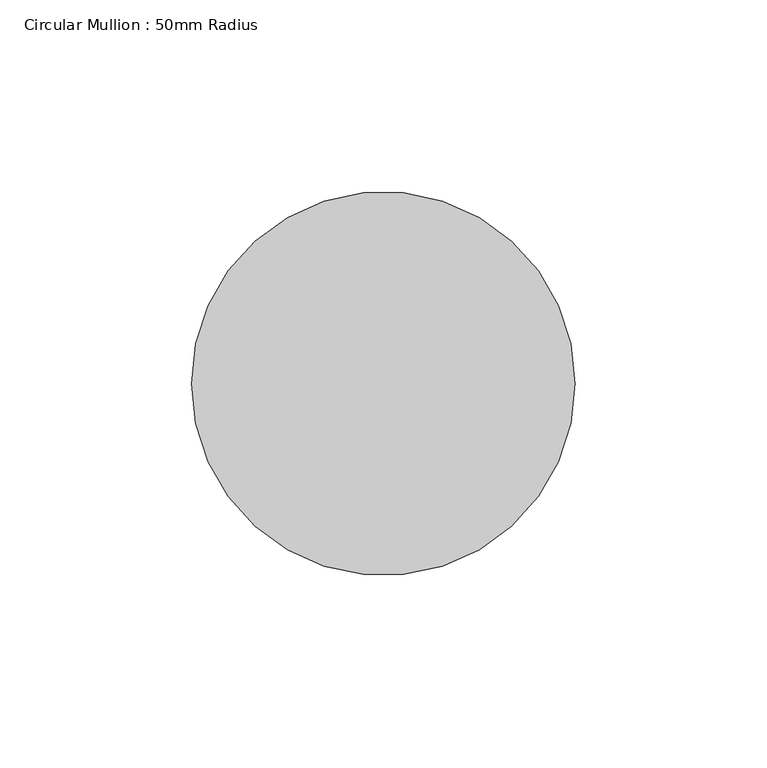
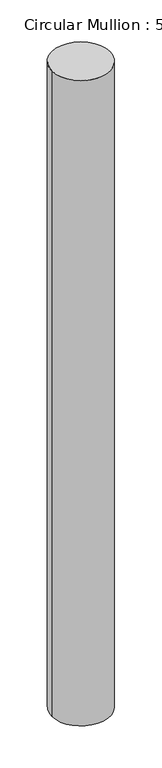
"""IFC4 building model written with IfcOpenShell, lengths in millimetres: member geometry, Circular Mullion : 50mm Radius."""

from ifc_helpers import new_model, si_unit, point, frame, origin, origin_2d, place, context, project, spatial, circle_curve, trimmed, segment, composite_curve, outline, extrude, source, transform, mapped, element, save


def circular_mullion_50mm_radius_569d8a70(model_context):
    return source(origin(), model_context, "Body", "SweptSolid", [
        extrude(outline(composite_curve([segment(trimmed(circle_curve(origin_2d(), 50.0), [point((50.0, 0.0))], [point((-50.0, 0.0))], False, "CARTESIAN"), True, "CONTINUOUS"), segment(trimmed(circle_curve(origin_2d(), 50.0), [point((-50.0, 0.0))], [point((50.0, 0.0))], False, "CARTESIAN"), True, "CONTINUOUS")], self_intersect=False)), frame((0.0, 0.0, -1170.1753315), z_axis=(0.0, 0.0, 1.0), x_axis=(1.0, 0.0, 0.0)), (0.0, 0.0, 1.0), 1170.1753315),
    ])


if __name__ == "__main__":
    model = new_model("IFC4")
    model_context = context("Model", 3, world=origin())
    ifc_project = project(units=[si_unit("LENGTHUNIT", "METRE", prefix="MILLI")], contexts=[model_context])
    site = spatial("IfcSite", under=ifc_project)
    building = spatial("IfcBuilding", under=site)
    placement = place(None, origin())
    circular_mullion_50mm_radius_shape = circular_mullion_50mm_radius_569d8a70(model_context)
    element("IfcMember", 1, ObjectType="Circular Mullion : 50mm Radius", at=placement, inside=building, context=model_context, shape_type="MappedRepresentation", body=[
        mapped(circular_mullion_50mm_radius_shape, transform((0.0, 0.0, 0.0), x_axis=(1.0, 0.0, 0.0), y_axis=(0.0, 1.0, 0.0), z_axis=(0.0, 0.0, 1.0))),
    ])
    save(model, "model.ifc")

# Revit data of these elements
# Type "Circular Mullion : 50mm Radius"
#   built-in parameter 1007350 = 0.164042 (stored number, unit not read)
# Element 1 (IfcMember, "Circular Mullion : 50mm Radius")
#   Materials on its faces: "Aluminium"
# Materials
#   "Aluminium": class "Metal", colour RGB 247 247 247, transparency 0, Description = "Aluminium 6061", Cost = 0
